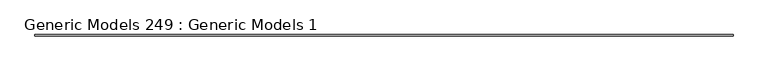
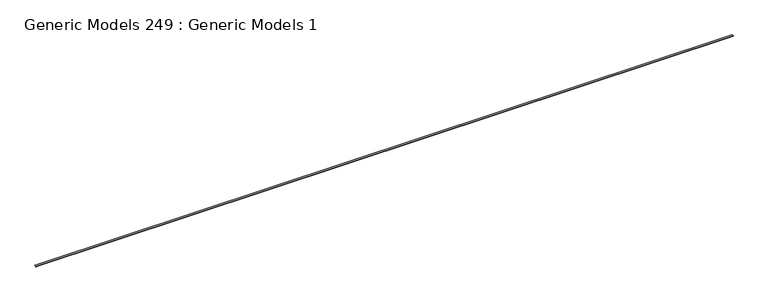
"""IFC4 building model written with IfcOpenShell, lengths in millimetres: proxy geometry, Generic Models 249 : Generic Models 1."""

from ifc_helpers import new_model, si_unit, origin, place, context, project, spatial, faceted_brep, source, transform, mapped, element, save


def generic_models_249_generic_models_1_f155bf51(model_context):
    return source(origin(), model_context, "Body", "Brep", [
        faceted_brep([(-5248.1628079, -20261.4171024, 126780.671), (-5248.1628079, -20261.4171024, 126802.896), (-5248.1628079, -20223.3171024, 126802.896), (-5248.1628079, -20223.3171024, 126801.626), (-5248.1628079, -20260.1471024, 126801.626), (-5248.1628079, -20260.1471024, 126781.941), (-5248.1628079, -20257.9373024, 126781.941), (-5248.1628079, -20257.9373024, 126783.6734564), (-5248.1628079, -20256.6673024, 126783.6734564), (-5248.1628079, -20256.6673024, 126780.671), (13801.8371921, -20261.4171024, 126780.671), (13801.8371921, -20256.6673024, 126780.671), (13801.8371921, -20256.6673024, 126783.6734564), (13801.8371921, -20257.9373024, 126783.6734564), (13801.8371921, -20257.9373024, 126781.941), (13801.8371921, -20260.1471024, 126781.941), (13801.8371921, -20260.1471024, 126801.626), (13801.8371921, -20223.3171024, 126801.626), (13801.8371921, -20223.3171024, 126802.896), (13801.8371921, -20261.4171024, 126802.896), (13593.8187142, -20223.3171024, 126802.896), (-5049.7812858, -20223.3171024, 126802.896), (13593.8187142, -20223.3171024, 126801.626), (-5049.7812858, -20223.3171024, 126801.626), (13593.8187142, -20260.1471024, 126801.626), (-5049.7812858, -20260.1471024, 126801.626), (13593.8187142, -20260.1471024, 126781.941), (-5049.7812858, -20260.1471024, 126781.941), (13593.8187142, -20257.9373024, 126781.941), (-5049.7812858, -20257.9373024, 126781.941), (-5049.7812858, -20257.9373024, 126783.6734564), (13593.8187142, -20257.9373024, 126783.6734564), (13593.8187142, -20256.6673024, 126783.6734564), (-5049.7812858, -20256.6673024, 126783.6734564), (13593.8187142, -20256.6673024, 126780.671), (-5049.7812858, -20256.6673024, 126780.671)], [[[0, 1, 2, 3, 4, 5, 6, 7, 8, 9]], [[10, 11, 12, 13, 14, 15, 16, 17, 18, 19]], [[1, 0, 10, 19]], [[2, 1, 19, 18, 20, 21]], [[3, 2, 21, 20, 18, 17, 22, 23]], [[4, 3, 23, 22, 17, 16, 24, 25]], [[5, 4, 25, 24, 16, 15, 26, 27]], [[6, 5, 27, 26, 15, 14, 28, 29]], [[8, 7, 30, 31, 13, 12, 32, 33]], [[9, 8, 33, 32, 12, 11, 34, 35]], [[0, 9, 35, 34, 11, 10]], [[7, 6, 29, 28, 14, 13, 31, 30]]]),
    ])


if __name__ == "__main__":
    model = new_model("IFC4")
    model_context = context("Model", 3, world=origin())
    ifc_project = project(units=[si_unit("LENGTHUNIT", "METRE", prefix="MILLI")], contexts=[model_context])
    site = spatial("IfcSite", under=ifc_project)
    building = spatial("IfcBuilding", under=site)
    placement = place(None, origin())
    generic_models_249_generic_models_1_shape = generic_models_249_generic_models_1_f155bf51(model_context)
    element("IfcBuildingElementProxy", 1, Name="Generic Models 249 : Generic Models 1", ObjectType="Generic Models 249 : Generic Models 1", at=placement, inside=building, context=model_context, shape_type="MappedRepresentation", body=[
        mapped(generic_models_249_generic_models_1_shape, transform((0.0, 0.0, 0.0), x_axis=(1.0, 0.0, 0.0), y_axis=(0.0, 1.0, 0.0), z_axis=(0.0, 0.0, 1.0))),
    ])
    save(model, "model.ifc")

# Revit data of these elements
# Element 1 (IfcBuildingElementProxy, "Generic Models 249 : Generic Models 1")
#   Materials on its faces: "_CONTINUOUS 16 GA. COPPER  J BEAD"
# Materials
#   "_CONTINUOUS 16 GA. COPPER  J BEAD": class "Generic", colour RGB 253 192 103, transparency 0, Cost = 0
